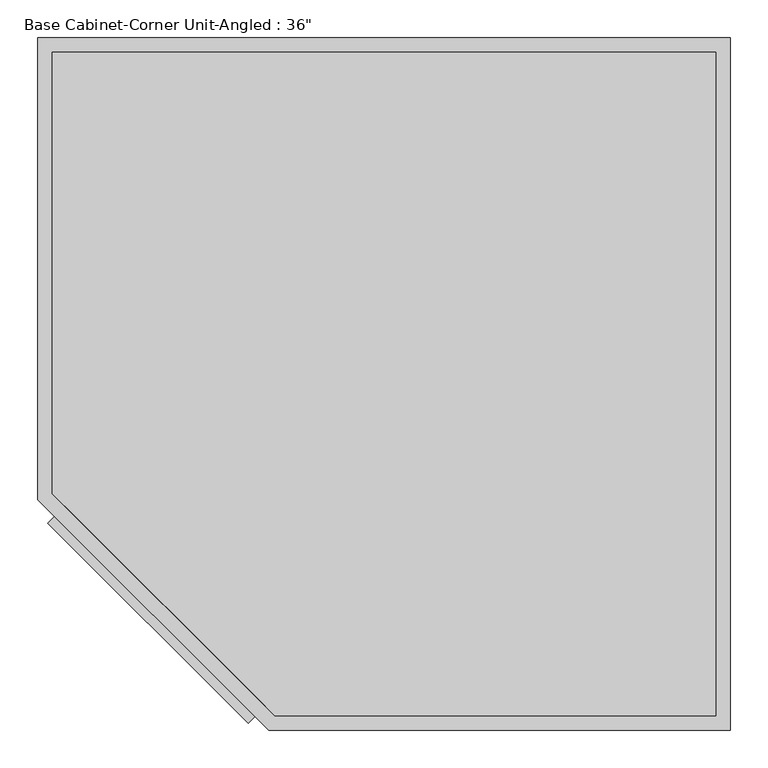
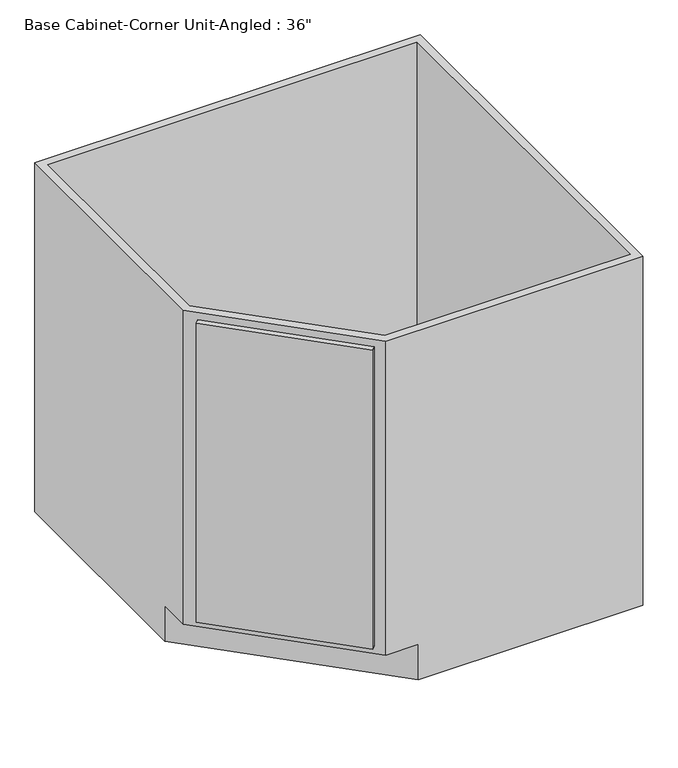
"""IFC4 building model written with IfcOpenShell, lengths in millimetres: furniture geometry."""

from ifc_helpers import new_model, si_unit, frame, origin, place, context, project, spatial, polyline, outline, extrude, faceted_brep, source, transform, mapped, element, save


def furniture_bfd559e3(model_context):
    return source(origin(), model_context, "Body", "SolidModel", [
        extrude(outline(polyline([(-109.5319116, -905.7284105), (-374.7303593, -641.0922321), (-352.3035566, -618.6177794), (-87.105109, -883.2539578), (-109.5319116, -905.7284105)])), frame((0.0, 0.0, 107.95), z_axis=(0.0, 0.0, 1.0), x_axis=(1.0, 0.0, 0.0)), (0.0, 0.0, 1.0), 749.3),
        faceted_brep([(526.7377049, 0.0, 876.3), (-387.6622951, 0.0, 876.3), (-387.6622951, -610.2462317, 876.3), (-82.8622951, -914.4, 876.3), (526.7377049, -914.4, 876.3), (-368.6122951, -602.3436184, 876.3), (-368.6122951, -19.05, 876.3), (507.6877049, -19.05, 876.3), (507.6877049, -895.35, 876.3), (-74.9833665, -895.35, 876.3), (-6.6622951, -914.4, 88.9), (-82.8622951, -914.4, 88.9), (-387.6622951, -610.2462317, 88.9), (-387.6622951, -534.0223805, 88.9), (-368.6122951, -553.0412615, 88.9), (-368.6122951, -602.3436184, 88.9), (-74.9833665, -895.35, 88.9), (-25.743465, -895.35, 88.9), (526.7377049, 0.0, 0.0), (-387.6622951, 0.0, 0.0), (-387.6622951, -534.0223805, 0.0), (-368.6122951, -19.05, 88.9), (507.6877049, -19.05, 88.9), (507.6877049, -895.35, 88.9), (-6.6622951, -914.4, 0.0), (526.7377049, -914.4, 0.0), (-100.5611906, -896.7386294, 857.25), (-100.5611906, -896.7386294, 107.95), (-365.7596382, -632.102451, 107.95), (-365.7596382, -632.102451, 857.25), (-87.105109, -883.2539578, 107.95), (-87.105109, -883.2539578, 857.25), (-352.3035566, -618.6177794, 857.25), (-352.3035566, -618.6177794, 107.95)], [[[0, 1, 2, 3, 4], [5, 6, 7, 8, 9]], [[10, 11, 12, 13, 14, 15, 16, 17]], [[1, 0, 18, 19]], [[2, 1, 19, 20, 13, 12]], [[6, 5, 15, 14, 21]], [[7, 6, 21, 22]], [[8, 7, 22, 23]], [[9, 8, 23, 17, 16]], [[4, 3, 11, 10, 24, 25]], [[0, 4, 25, 18]], [[14, 17, 23, 22, 21]], [[18, 25, 24, 20, 19]], [[20, 24, 10, 17, 14, 13]], [[3, 2, 12, 11], [26, 27, 28, 29]], [[5, 9, 16, 15], [30, 31, 32, 33]], [[30, 27, 26, 31]], [[27, 30, 33, 28]], [[28, 33, 32, 29]], [[31, 26, 29, 32]]]),
        extrude(outline(polyline([(507.6877049, -19.05), (507.6877049, -895.35), (-74.9833665, -895.35), (-368.6122951, -602.3436184), (-368.6122951, -19.05), (507.6877049, -19.05)])), frame((0.0, 0.0, 88.9), z_axis=(0.0, 0.0, 1.0), x_axis=(1.0, 0.0, 0.0)), (0.0, 0.0, 1.0), 19.05),
    ])


if __name__ == "__main__":
    model = new_model("IFC4")
    model_context = context("Model", 3, world=origin())
    ifc_project = project(units=[si_unit("LENGTHUNIT", "METRE", prefix="MILLI")], contexts=[model_context])
    site = spatial("IfcSite", under=ifc_project)
    building = spatial("IfcBuilding", under=site)
    placement = place(None, origin())
    furniture_shape = furniture_bfd559e3(model_context)
    element("IfcFurniture", 1, ObjectType="Base Cabinet-Corner Unit-Angled : 36\"", at=placement, inside=building, context=model_context, shape_type="MappedRepresentation", body=[
        mapped(furniture_shape, transform((0.0, 0.0, 0.0), x_axis=(1.0, 0.0, 0.0), y_axis=(0.0, 1.0, 0.0), z_axis=(0.0, 0.0, 1.0))),
    ])
    save(model, "model.ifc")

# Revit data of these elements
# Type "Base Cabinet-Corner Unit-Angled : 36\""
#   Assembly Code = "C1030410"
#   Depth = 3' - 0"
#   Height = 2' - 10 1/2"
#   Toe Height = 0' - 3 1/2"
#   Width = 3' - 0"
#   Cabinet Material = none
#   Door/Drawer Material = none
# Element 1 (IfcFurniture, "Base Cabinet-Corner Unit-Angled : 36\"")
#   Materials on its faces: "Cabinets"
# Materials
#   "Cabinets": class "Miscellaneous", colour RGB 249 249 249, transparency 0
